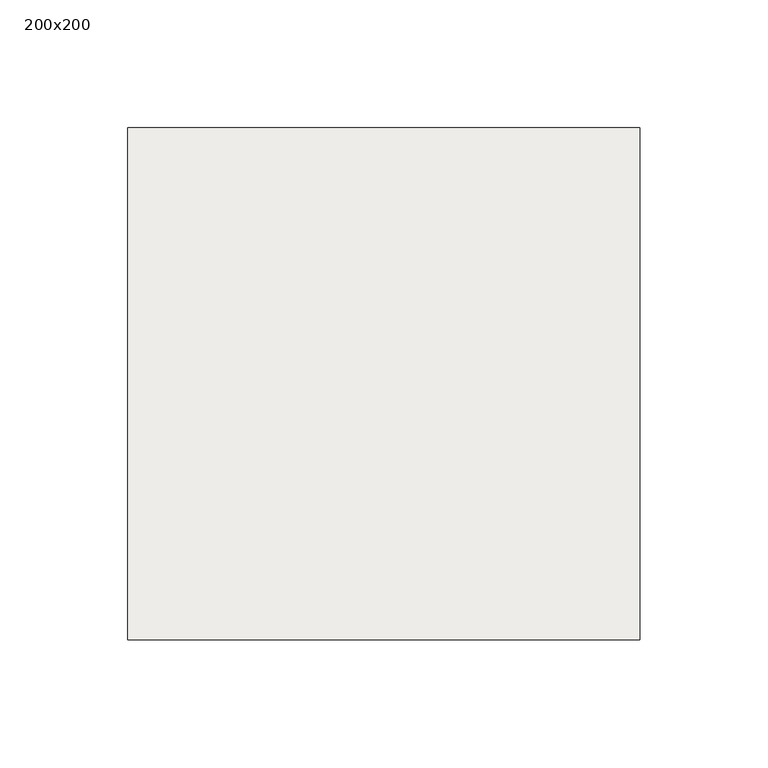
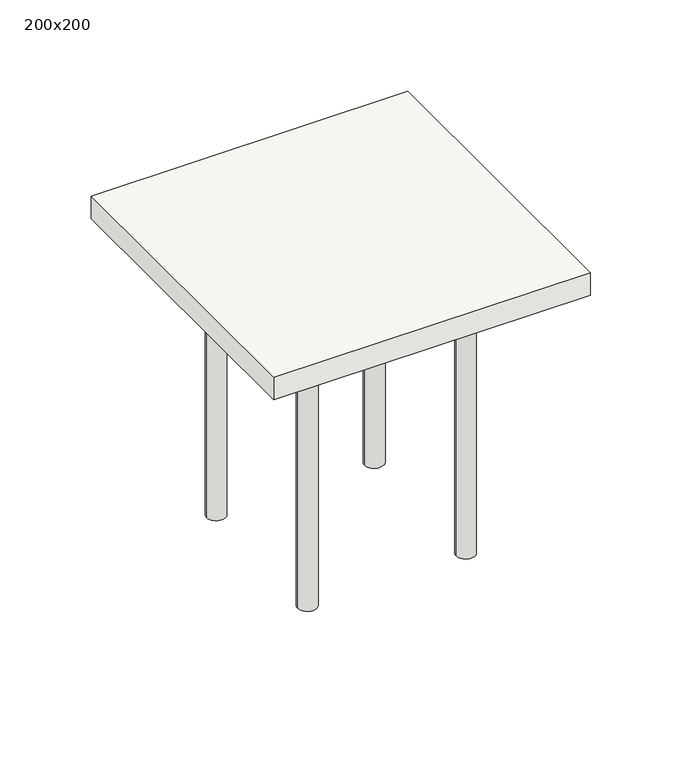
"""IFC4 building model written with IfcOpenShell, lengths in millimetres: slab geometry, Innstøpningsplate : 200x200."""

from ifc_helpers import new_model, si_unit, point, frame, frame_2d, origin, place, context, project, spatial, polyline, circle_curve, trimmed, segment, composite_curve, outline, extrude, source, transform, mapped, element, save


def slab_200x200_02b47a6d(model_context):
    return source(origin(), model_context, "Body", "SweptSolid", [
        extrude(outline(composite_curve([segment(trimmed(circle_curve(frame_2d((269.1096391, -214.6158832)), 6.0), [point((263.1096391, -214.6158832))], [point((275.1096391, -214.6158832))], False, "CARTESIAN"), True, "CONTINUOUS"), segment(trimmed(circle_curve(frame_2d((269.1096391, -214.6158832)), 6.0), [point((275.1096391, -214.6158832))], [point((263.1096391, -214.6158832))], False, "CARTESIAN"), True, "CONTINUOUS")], self_intersect=False)), frame((0.0, 0.0, -200.0), z_axis=(0.0, 0.0, 1.0), x_axis=(1.0, 0.0, 0.0)), (0.0, 0.0, 1.0), 185.0),
        extrude(outline(composite_curve([segment(trimmed(circle_curve(frame_2d((369.1096391, -214.6158832)), 6.0), [point((363.1096391, -214.6158832))], [point((375.1096391, -214.6158832))], False, "CARTESIAN"), True, "CONTINUOUS"), segment(trimmed(circle_curve(frame_2d((369.1096391, -214.6158832)), 6.0), [point((375.1096391, -214.6158832))], [point((363.1096391, -214.6158832))], False, "CARTESIAN"), True, "CONTINUOUS")], self_intersect=False)), frame((0.0, 0.0, -200.0), z_axis=(0.0, 0.0, 1.0), x_axis=(1.0, 0.0, 0.0)), (0.0, 0.0, 1.0), 185.0),
        extrude(outline(composite_curve([segment(trimmed(circle_curve(frame_2d((369.1096391, -314.6158832)), 6.0), [point((363.1096391, -314.6158832))], [point((375.1096391, -314.6158832))], False, "CARTESIAN"), True, "CONTINUOUS"), segment(trimmed(circle_curve(frame_2d((369.1096391, -314.6158832)), 6.0), [point((375.1096391, -314.6158832))], [point((363.1096391, -314.6158832))], False, "CARTESIAN"), True, "CONTINUOUS")], self_intersect=False)), frame((0.0, 0.0, -200.0), z_axis=(0.0, 0.0, 1.0), x_axis=(1.0, 0.0, 0.0)), (0.0, 0.0, 1.0), 185.0),
        extrude(outline(composite_curve([segment(trimmed(circle_curve(frame_2d((269.1096391, -314.6158832)), 6.0), [point((263.1096391, -314.6158832))], [point((275.1096391, -314.6158832))], False, "CARTESIAN"), True, "CONTINUOUS"), segment(trimmed(circle_curve(frame_2d((269.1096391, -314.6158832)), 6.0), [point((275.1096391, -314.6158832))], [point((263.1096391, -314.6158832))], False, "CARTESIAN"), True, "CONTINUOUS")], self_intersect=False)), frame((0.0, 0.0, -200.0), z_axis=(0.0, 0.0, 1.0), x_axis=(1.0, 0.0, 0.0)), (0.0, 0.0, 1.0), 185.0),
        extrude(outline(polyline([(419.1096391, -164.6158832), (419.1096391, -364.6158832), (219.1096391, -364.6158832), (219.1096391, -164.6158832), (419.1096391, -164.6158832)])), frame((0.0, 0.0, -15.0), z_axis=(0.0, 0.0, 1.0), x_axis=(1.0, 0.0, 0.0)), (0.0, 0.0, 1.0), 15.0),
    ])


if __name__ == "__main__":
    model = new_model("IFC4")
    model_context = context("Model", 3, world=origin())
    ifc_project = project(units=[si_unit("LENGTHUNIT", "METRE", prefix="MILLI")], contexts=[model_context])
    site = spatial("IfcSite", under=ifc_project)
    building = spatial("IfcBuilding", under=site)
    placement = place(None, origin())
    slab_200x200_shape = slab_200x200_02b47a6d(model_context)
    element("IfcSlab", 1, ObjectType="Innstøpningsplate : 200x200", at=placement, inside=building, context=model_context, shape_type="MappedRepresentation", body=[
        mapped(slab_200x200_shape, transform((0.0, 0.0, 0.0), x_axis=(1.0, 0.0, 0.0), y_axis=(0.0, 1.0, 0.0), z_axis=(0.0, 0.0, 1.0))),
    ])
    save(model, "model.ifc")

# Revit data of these elements
# Type "Innstøpningsplate : 200x200"
#   NS3457-8 Code = "BAD"
#   NS3451 Code = ""
#   NS3457-8 = "BAD Knutepunkt, innstøpningsgods"
#   NS3451 = ""
#   Manufacturer = "Norconsult"
#   T = 15 mm
#   H = 200 mm
#   Default Elevation = 1000 mm
#   B = 200 mm
#   Armering d = 200 mm
#   Armering b = 50 mm
#   Armering Radius = 6 mm
#   Armering Dia = 12 mm
#   Material Plate = Metal - Steel - 345 MPa
#   Material Armering = Metal - Steel - 345 MPa
#   Assembly Code = ""
# Element 1 (IfcSlab, "Innstøpningsplate : 200x200")
#   Materials on its faces: "Metal - Steel - 345 MPa"
# Materials
#   "Metal - Steel - 345 MPa": class "Unassigned", colour RGB 128 64 64, transparency 0, Description = "Steel 345 MPa"
